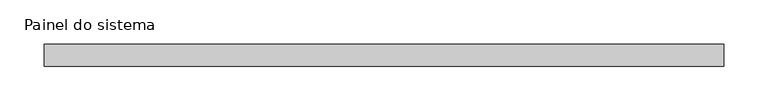
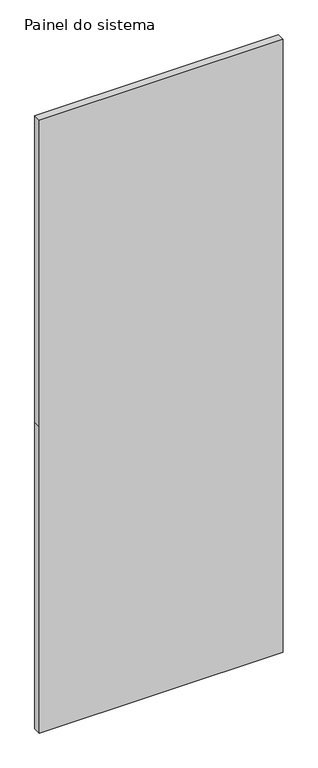
"""IFC4 building model written with IfcOpenShell, lengths in millimetres: plate geometry, Painel do sistema : Envidraçado."""

from ifc_helpers import new_model, si_unit, frame, origin, place, context, project, spatial, polyline, outline, extrude, source, transform, mapped, element, save


def painel_do_sistema_c7f0a930(model_context):
    return source(origin(), model_context, "Body", "SweptSolid", [
        extrude(outline(polyline([(0.0, -385.4916666), (0.0, 385.4916666), (1025.0, 385.4916666), (2050.0, 385.4916666), (2050.0, -385.4916666), (1025.0, -385.4916666), (0.0, -385.4916666)])), frame((0.0, -49.5, 0.0), z_axis=(0.0, 1.0, 0.0), x_axis=(0.0, 0.0, 1.0)), (0.0, 0.0, 1.0), 25.0),
    ])


if __name__ == "__main__":
    model = new_model("IFC4")
    model_context = context("Model", 3, world=origin())
    ifc_project = project(units=[si_unit("LENGTHUNIT", "METRE", prefix="MILLI")], contexts=[model_context])
    site = spatial("IfcSite", under=ifc_project)
    building = spatial("IfcBuilding", under=site)
    placement = place(None, origin())
    painel_do_sistema_shape = painel_do_sistema_c7f0a930(model_context)
    element("IfcPlate", 1, ObjectType="Painel do sistema : Envidraçado", at=placement, inside=building, context=model_context, shape_type="MappedRepresentation", body=[
        mapped(painel_do_sistema_shape, transform((0.0, 0.0, 0.0), x_axis=(1.0, 0.0, 0.0), y_axis=(0.0, 1.0, 0.0), z_axis=(0.0, 0.0, 1.0))),
    ])
    save(model, "model.ifc")

# Revit data of these elements
# Type "Painel do sistema : Envidraçado"
#   Construction Type Id = "GSP4R"
#   Analytic Construction = "Vidraça única Pilkington 1/8 pol"
#   Visual Light Transmittance = 0.9
#   Solar Heat Gain Coefficient = 0.86
#   Heat Transfer Coefficient (U) = 6.7069 W/(m²·K)
# Element 1 (IfcPlate, "Painel do sistema : Envidraçado")
#   Materials on its faces: ".VIDRO GENÉRICO"
# Materials
#   ".VIDRO GENÉRICO": class ".CC_VIDRO", colour RGB 0 128 192, transparency 0.9, Description = "Vidro comum", Cost = 0
